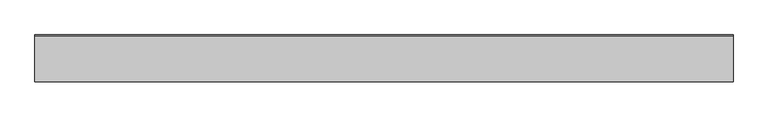
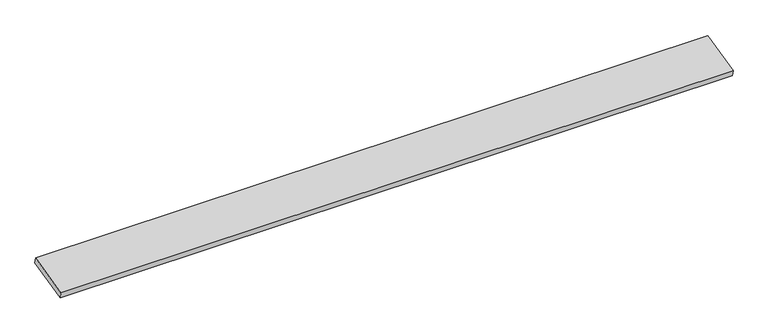
"""IFC4 building model written with IfcOpenShell, lengths in millimetres: proxy geometry, 1X WOODTRIM : 1X WOODTRIM."""

from ifc_helpers import new_model, si_unit, frame, origin, place, context, project, spatial, polyline, outline, extrude, source, transform, mapped, element, save


def generic_models_a2e2f502(model_context):
    return source(origin(), model_context, "Body", "SweptSolid", [
        extrude(outline(polyline([(0.0, -133.35), (0.0, 0.0), (2000.25, 0.0), (2000.25, -133.35), (0.0, -133.35)])), frame((12382.7678845, -5403.0837198, 42756.7494343), z_axis=(0.0, -0.23798663042445214, 0.9712684303215128), x_axis=(1.0, 0.0, 0.0)), (0.0, 0.0, 1.0), 19.05),
    ])


if __name__ == "__main__":
    model = new_model("IFC4")
    model_context = context("Model", 3, world=origin())
    ifc_project = project(units=[si_unit("LENGTHUNIT", "METRE", prefix="MILLI")], contexts=[model_context])
    site = spatial("IfcSite", under=ifc_project)
    building = spatial("IfcBuilding", under=site)
    placement = place(None, origin())
    generic_models_shape = generic_models_a2e2f502(model_context)
    element("IfcBuildingElementProxy", 1, Name="1X WOODTRIM : 1X WOODTRIM", ObjectType="1X WOODTRIM : 1X WOODTRIM", at=placement, inside=building, context=model_context, shape_type="MappedRepresentation", body=[
        mapped(generic_models_shape, transform((0.0, 0.0, 0.0), x_axis=(1.0, 0.0, 0.0), y_axis=(0.0, 1.0, 0.0), z_axis=(0.0, 0.0, 1.0))),
    ])
    save(model, "model.ifc")

# Revit data of these elements
# Type "1X WOODTRIM : 1X WOODTRIM"
#   NameOverride = "1X WOODTRIM"
# Element 1 (IfcBuildingElementProxy, "1X WOODTRIM : 1X WOODTRIM")
#   Materials on its faces: "1X WOOD TRIM AS REQUIRED"
# Materials
#   "1X WOOD TRIM AS REQUIRED": class "Unassigned", colour RGB 166 124 85, transparency 0
